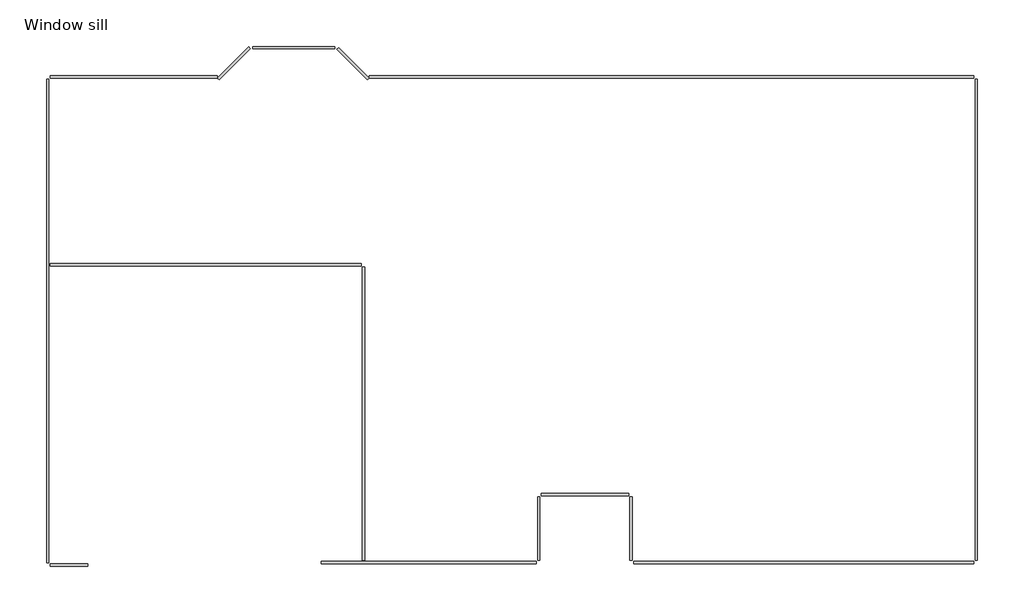
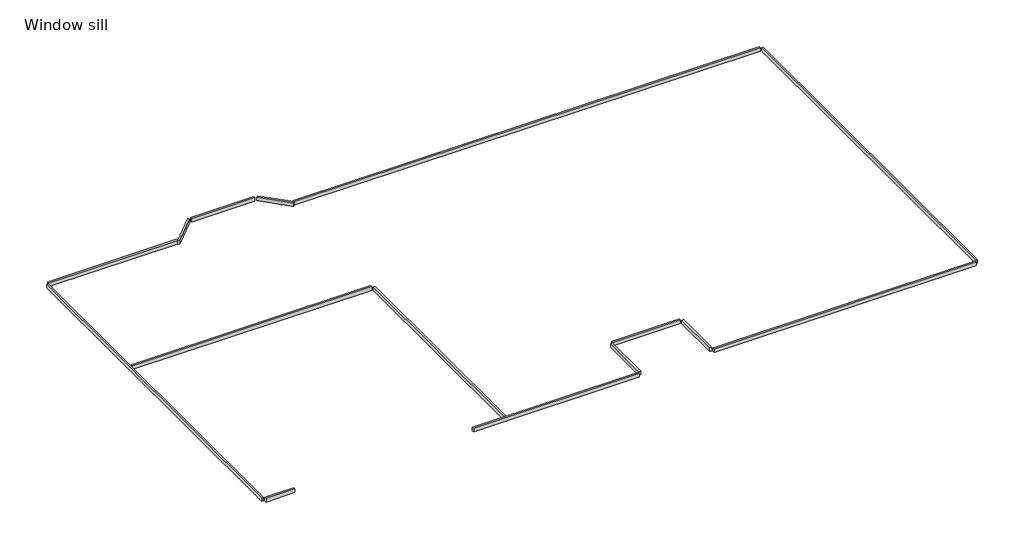
# One storey: 15 beams.
"""IFC4 building model written with IfcOpenShell, lengths in millimetres."""

import ifcopenshell
import ifcopenshell.guid

model = None  # the IFC model being written
_history = None  # IfcOwnerHistory: only IFC2X3 demands one
_inside = {}  # id of a spatial element -> (the spatial element, [elements in it])
_under = {}  # id of a project, library or spatial element -> (it, [spatial elements below it])
_declared = {}  # id of a project -> (the project, [libraries it declares])
_typed = {}  # id of a type object -> (the type object, [elements of that type])
_made_of = {}  # id of a material, layer set ... -> (it, [elements and type objects made of it])


def new_model(schema):
    """Start an empty IFC model of exactly this schema.

    Asked for "IFC4X3", IfcOpenShell would pick the latest addendum, in which some entities
    have other attributes; the version numbers below select the first issue.
    IFC2X3 requires an IfcOwnerHistory on every rooted entity: one is made here for all.
    """
    global model, _history
    if schema == "IFC4X3":
        model = ifcopenshell.file(schema_version=(4, 3, 0, 0))
    else:
        model = ifcopenshell.file(schema=schema)
    _inside.clear()
    _under.clear()
    _declared.clear()
    _typed.clear()
    _made_of.clear()
    _history = None
    if model.schema == "IFC2X3":
        org = make("IfcOrganization", Name="unknown")
        user = make(
            "IfcPersonAndOrganization",
            ThePerson=make("IfcPerson", FamilyName="unknown"),
            TheOrganization=org,
        )
        app = make(
            "IfcApplication",
            ApplicationDeveloper=org,
            Version="unknown",
            ApplicationFullName="unknown",
            ApplicationIdentifier="unknown",
        )
        _history = make(
            "IfcOwnerHistory",
            OwningUser=user,
            OwningApplication=app,
            ChangeAction="ADDED",
            CreationDate=0,
        )
    return model


def make(cls, **values):
    """One entity of the class cls with the attributes given. An attribute that is None is left unset."""
    return model.create_entity(
        cls, **{name: value for name, value in values.items() if value is not None}
    )


def rooted(cls, **values):
    """An entity with a GlobalId (a new one), such as an element, a storey or a relation."""
    return make(cls, GlobalId=ifcopenshell.guid.new(), OwnerHistory=_history, **values)


def si_unit(unit_type, name, prefix=None):
    """IfcSIUnit, for example si_unit("LENGTHUNIT", "METRE", prefix="MILLI")."""
    return make("IfcSIUnit", UnitType=unit_type, Prefix=prefix, Name=name)


def assignment(units):
    """IfcUnitAssignment: the units of a project."""
    return None if units is None else make("IfcUnitAssignment", Units=units)


def point(xyz):
    """IfcCartesianPoint."""
    return None if xyz is None else make("IfcCartesianPoint", Coordinates=xyz)


def direction(xyz):
    """IfcDirection."""
    return None if xyz is None else make("IfcDirection", DirectionRatios=xyz)


def frame(location, z_axis=None, x_axis=None):
    """IfcAxis2Placement3D, a coordinate frame: its origin and axes. An axis left out is left unset."""
    return make(
        "IfcAxis2Placement3D",
        Location=point(location),
        Axis=direction(z_axis),
        RefDirection=direction(x_axis),
    )


def origin():
    """The frame at (0, 0, 0) with its axes left unset."""
    return frame((0.0, 0.0, 0.0))


def place(relative_to, where):
    """IfcLocalPlacement: puts the frame where relative to a parent placement (None: the world)."""
    return make(
        "IfcLocalPlacement", PlacementRelTo=relative_to, RelativePlacement=where
    )


def context(
    kind, dimensions, precision=None, world=None, true_north=None, identifier=None
):
    """IfcGeometricRepresentationContext, for example the 3D "Model" context."""
    return make(
        "IfcGeometricRepresentationContext",
        ContextIdentifier=identifier,
        ContextType=kind,
        CoordinateSpaceDimension=dimensions,
        Precision=precision,
        WorldCoordinateSystem=world,
        TrueNorth=true_north,
    )


def project(units=None, contexts=None):
    """IfcProject with its units and contexts."""
    return rooted(
        "IfcProject",
        Name="project",
        RepresentationContexts=contexts,
        UnitsInContext=assignment(units),
    )


def spatial(cls, under=None, at=None, **own):
    """A site, building, storey or space (cls), placed at a placement, below another one or the project."""
    s = rooted(cls, ObjectPlacement=at, **own)
    if under is not None:
        _under.setdefault(under.id(), (under, []))[1].append(s)
    return s


def polyline(points):
    """IfcPolyline through the points."""
    return make("IfcPolyline", Points=[point(p) for p in points])


def outline(outer, holes=None, kind="AREA"):
    """IfcArbitraryClosedProfileDef: a profile drawn as a closed curve; with holes, ...WithVoids."""
    if holes is None:
        return make("IfcArbitraryClosedProfileDef", ProfileType=kind, OuterCurve=outer)
    return make(
        "IfcArbitraryProfileDefWithVoids",
        ProfileType=kind,
        OuterCurve=outer,
        InnerCurves=holes,
    )


def extrude(swept, where, along, depth):
    """IfcExtrudedAreaSolid: the profile swept, set in the frame where, extruded along a direction by depth."""
    return make(
        "IfcExtrudedAreaSolid",
        SweptArea=swept,
        Position=where,
        ExtrudedDirection=direction(along),
        Depth=depth,
    )


def shape(context_of_items, identifier, shape_type, items):
    """IfcShapeRepresentation: the items that make up one representation, for example the "Body"."""
    return make(
        "IfcShapeRepresentation",
        ContextOfItems=context_of_items,
        RepresentationIdentifier=identifier,
        RepresentationType=shape_type,
        Items=items,
    )


def source(mapping_origin, context_of_items, identifier, shape_type, items):
    """IfcRepresentationMap: a shape defined once, which mapped items show again and again."""
    return make(
        "IfcRepresentationMap",
        MappingOrigin=mapping_origin,
        MappedRepresentation=shape(context_of_items, identifier, shape_type, items),
    )


def transform(
    local_origin,
    x_axis=None,
    y_axis=None,
    z_axis=None,
    scale=None,
    scale2=None,
    scale3=None,
    uniform=True,
):
    """IfcCartesianTransformationOperator3D, or its non-uniform kind. x_axis, y_axis, z_axis: its Axis1, 2, 3."""
    if uniform:
        return make(
            "IfcCartesianTransformationOperator3D",
            Axis1=direction(x_axis),
            Axis2=direction(y_axis),
            LocalOrigin=point(local_origin),
            Scale=scale,
            Axis3=direction(z_axis),
        )
    return make(
        "IfcCartesianTransformationOperator3DnonUniform",
        Axis1=direction(x_axis),
        Axis2=direction(y_axis),
        LocalOrigin=point(local_origin),
        Scale=scale,
        Axis3=direction(z_axis),
        Scale2=scale2,
        Scale3=scale3,
    )


def mapped(mapping_source, mapping_target):
    """IfcMappedItem: shows the shape of a source again, moved by a transform."""
    return make(
        "IfcMappedItem", MappingSource=mapping_source, MappingTarget=mapping_target
    )


def made_of(thing, what):
    """Note that an element or type object is made of a material, layer set ...; save() writes the relation."""
    if what is not None:
        _made_of.setdefault(what.id(), (what, []))[1].append(thing)
    return thing


def element(
    cls,
    number,
    at=None,
    inside=None,
    cuts=None,
    type_object=None,
    material=None,
    context=None,
    identifier="Body",
    shape_type=None,
    held_by="IfcProductDefinitionShape",
    body=None,
    shapes=None,
    **own,
):
    """One element of the class cls, such as IfcWall. Its Tag is "e" and its number.

    at: its placement. inside: the storey or other place that contains it. cuts: it is an
    opening in that element (IfcRelVoidsElement). A single representation is given by context,
    identifier, shape_type and body (its items); several are given by shapes. held_by: the class
    of the entity that holds the representations. save() writes the other relations.
    """
    e = rooted(cls, Tag="e%d" % number, ObjectPlacement=at, **own)
    if body is not None:
        shapes = [shape(context, identifier, shape_type, body)]
    if shapes is not None:
        e.Representation = make(held_by, Representations=shapes)
    if inside is not None:
        _inside.setdefault(inside.id(), (inside, []))[1].append(e)
    if cuts is not None:
        rooted(
            "IfcRelVoidsElement", RelatingBuildingElement=cuts, RelatedOpeningElement=e
        )
    if type_object is not None:
        _typed.setdefault(type_object.id(), (type_object, []))[1].append(e)
    return made_of(e, material)


def aggregate(whole, parts):
    """IfcRelAggregates: a whole, such as a stair, and the parts it consists of."""
    return rooted("IfcRelAggregates", RelatingObject=whole, RelatedObjects=parts)


def save(model, path):
    """Write the relations noted so far, then the file.

    IfcRelAggregates (storeys below a building ...), IfcRelContainedInSpatialStructure (elements
    in a storey), IfcRelDefinesByType, IfcRelAssociatesMaterial and IfcRelDeclares: one each for
    every whole, place, type object, material and project.
    """
    for whole, parts in _under.values():
        aggregate(whole, parts)
    for where, things in _inside.values():
        rooted(
            "IfcRelContainedInSpatialStructure",
            RelatedElements=things,
            RelatingStructure=where,
        )
    for kind, things in _typed.values():
        rooted("IfcRelDefinesByType", RelatedObjects=things, RelatingType=kind)
    for what, things in _made_of.values():
        rooted("IfcRelAssociatesMaterial", RelatedObjects=things, RelatingMaterial=what)
    for by, libraries in _declared.values():
        rooted("IfcRelDeclares", RelatingContext=by, RelatedDefinitions=libraries)
    model.write(path)


def beam_717df711(model_context):
    return source(origin(), model_context, "Body", "SweptSolid", [
        extrude(outline(polyline([(1716.6789755, 25.4), (1716.6789755, -25.4), (-1777.9999994, -25.4), (-1777.9999994, 25.4), (1716.6789755, 25.4)])), frame((0.0, 0.0, -50.8), z_axis=(0.0, 0.0, 1.0), x_axis=(1.0, 0.0, 0.0)), (0.0, 0.0, 1.0), 101.6),
    ])


def beam_0fe92c09(model_context):
    return source(origin(), model_context, "Body", "SweptSolid", [
        extrude(outline(polyline([(431.690501, 25.4), (431.690501, -25.4), (-492.3733183, -25.4), (-492.3733183, 25.4), (431.690501, 25.4)])), frame((0.0, 0.0, -50.8), z_axis=(0.0, 0.0, 1.0), x_axis=(1.0, 0.0, 0.0)), (0.0, 0.0, 1.0), 101.6),
    ])


def beam_3500c81b(model_context):
    return source(origin(), model_context, "Body", "SweptSolid", [
        extrude(outline(polyline([(863.6, 25.4), (863.6, -25.4), (-845.1882072, -25.4), (-845.1882072, 25.4), (863.6, 25.4)])), frame((0.0, 0.0, -50.8), z_axis=(0.0, 0.0, 1.0), x_axis=(1.0, 0.0, 0.0)), (0.0, 0.0, 1.0), 101.6),
    ])


def beam_4e9e3d70(model_context):
    return source(origin(), model_context, "Body", "SweptSolid", [
        extrude(outline(polyline([(492.3733183, 25.4), (492.3733183, -25.4), (-405.6522938, -25.4), (-405.6522938, 25.4), (492.3733183, 25.4)])), frame((0.0, 0.0, -50.8), z_axis=(0.0, 0.0, 1.0), x_axis=(1.0, 0.0, 0.0)), (0.0, 0.0, 1.0), 101.6),
    ])


def beam_5a8d2df6(model_context):
    return source(origin(), model_context, "Body", "SweptSolid", [
        extrude(outline(polyline([(6349.9999994, 25.4), (6349.9999994, -25.4), (-6288.6789755, -25.4), (-6288.6789755, 25.4), (6349.9999994, 25.4)])), frame((0.0, 0.0, -50.8), z_axis=(0.0, 0.0, 1.0), x_axis=(1.0, 0.0, 0.0)), (0.0, 0.0, 1.0), 101.6),
    ])


def beam_8dd97a7c(model_context):
    return source(origin(), model_context, "Body", "SweptSolid", [
        extrude(outline(polyline([(5029.1999994, 25.4), (5029.1999994, -25.4), (-5029.1999994, -25.4), (-5029.1999994, 25.4), (5029.1999994, 25.4)])), frame((0.0, 0.0, -50.8), z_axis=(0.0, 0.0, 1.0), x_axis=(1.0, 0.0, 0.0)), (0.0, 0.0, 1.0), 101.6),
    ])


def beam_44bcd8c2(model_context):
    return source(origin(), model_context, "Body", "SweptSolid", [
        extrude(outline(polyline([(3555.9999994, 25.4), (3555.9999994, -25.4), (-3555.9999994, -25.4), (-3555.9999994, 25.4), (3555.9999994, 25.4)])), frame((0.0, 0.0, -50.8), z_axis=(0.0, 0.0, 1.0), x_axis=(1.0, 0.0, 0.0)), (0.0, 0.0, 1.0), 101.6),
    ])


def beam_ec20356b(model_context):
    return source(origin(), model_context, "Body", "SweptSolid", [
        extrude(outline(polyline([(660.3999994, 25.4), (660.3999994, -25.4), (-660.3999994, -25.4), (-660.3999994, 25.4), (660.3999994, 25.4)])), frame((0.0, 0.0, -50.8), z_axis=(0.0, 0.0, 1.0), x_axis=(1.0, 0.0, 0.0)), (0.0, 0.0, 1.0), 101.6),
    ])


def beam_17170791(model_context):
    return source(origin(), model_context, "Body", "SweptSolid", [
        extrude(outline(polyline([(914.3999994, 25.4), (914.3999994, -25.4), (-914.3999994, -25.4), (-914.3999994, 25.4), (914.3999994, 25.4)])), frame((0.0, 0.0, -50.8), z_axis=(0.0, 0.0, 1.0), x_axis=(1.0, 0.0, 0.0)), (0.0, 0.0, 1.0), 101.6),
    ])


def beam_5c93efd5(model_context):
    return source(origin(), model_context, "Body", "SweptSolid", [
        extrude(outline(polyline([(3063.8749994, 25.4), (3063.8749994, -25.4), (-3063.8749994, -25.4), (-3063.8749994, 25.4), (3063.8749994, 25.4)])), frame((0.0, 0.0, -50.8), z_axis=(0.0, 0.0, 1.0), x_axis=(1.0, 0.0, 0.0)), (0.0, 0.0, 1.0), 101.6),
    ])


def beam_4ff5e491(model_context):
    return source(origin(), model_context, "Body", "SweptSolid", [
        extrude(outline(polyline([(3248.0249994, 25.4), (3248.0249994, -25.4), (-3248.0249994, -25.4), (-3248.0249994, 25.4), (3248.0249994, 25.4)])), frame((0.0, 0.0, -50.8), z_axis=(0.0, 0.0, 1.0), x_axis=(1.0, 0.0, 0.0)), (0.0, 0.0, 1.0), 101.6),
    ])


def beam_8f11d8aa(model_context):
    return source(origin(), model_context, "Body", "SweptSolid", [
        extrude(outline(polyline([(5054.5999994, 25.4), (5054.5999994, -25.4), (-5054.5999994, -25.4), (-5054.5999994, 25.4), (5054.5999994, 25.4)])), frame((0.0, 0.0, -50.8), z_axis=(0.0, 0.0, 1.0), x_axis=(1.0, 0.0, 0.0)), (0.0, 0.0, 1.0), 101.6),
    ])


def beam_175a3536(model_context):
    return source(origin(), model_context, "Body", "SweptSolid", [
        extrude(outline(polyline([(2249.4875, 25.4), (2249.4875, -25.4), (-2249.4874994, -25.4), (-2249.4874994, 25.4), (2249.4875, 25.4)])), frame((0.0, 0.0, -50.8), z_axis=(0.0, 0.0, 1.0), x_axis=(1.0, 0.0, 0.0)), (0.0, 0.0, 1.0), 101.6),
    ])


def beam_ce158ae4(model_context):
    return source(origin(), model_context, "Body", "SweptSolid", [
        extrude(outline(polyline([(392.1124994, 25.4), (392.1124994, -25.4), (-392.1125, -25.4), (-392.1125, 25.4), (392.1124994, 25.4)])), frame((0.0, 0.0, -50.8), z_axis=(0.0, 0.0, 1.0), x_axis=(1.0, 0.0, 0.0)), (0.0, 0.0, 1.0), 101.6),
    ])


model = new_model("IFC4")

# Units and contexts
model_context = context("Model", 3, world=origin())
ifc_project = project(units=[si_unit("LENGTHUNIT", "METRE", prefix="MILLI")], contexts=[model_context])

# Site, building, storey
site = spatial("IfcSite", under=ifc_project)
building = spatial("IfcBuilding", under=site)
storey = spatial("IfcBuildingStorey", under=building, Name="Window sill", Elevation=1168.4)

# Beams
placement = place(None, origin())
beam_shape = beam_717df711(model_context)
element("IfcBeam", 1, ObjectType="Dimension Lumber : BLDG 6241 2X4\" TRUSS MEMBER", at=placement, inside=storey, context=model_context, shape_type="MappedRepresentation", body=[
    mapped(beam_shape, transform((-15921.614829, 5156.9284114, 1117.6), x_axis=(1.0, 0.0, 0.0), y_axis=(0.0, 1.0, 0.0), z_axis=(0.0, 0.0, 1.0))),
])
beam_2_shape = beam_0fe92c09(model_context)
element("IfcBeam", 2, ObjectType="Dimension Lumber : BLDG 6241 2X4\" TRUSS MEMBER", at=placement, inside=storey, context=model_context, shape_type="MappedRepresentation", body=[
    mapped(beam_2_shape, transform((-13838.814829, 5461.7284114, 1117.6), x_axis=(0.7071067811865481, 0.7071067811865468, 0.0), y_axis=(-0.7071067811865468, 0.7071067811865481, 0.0), z_axis=(0.0, 0.0, 1.0))),
])
beam_3_shape = beam_3500c81b(model_context)
element("IfcBeam", 3, ObjectType="Dimension Lumber : BLDG 6241 2X4\" TRUSS MEMBER", at=placement, inside=storey, context=model_context, shape_type="MappedRepresentation", body=[
    mapped(beam_3_shape, transform((-12619.614829, 5766.5284114, 1117.6), x_axis=(1.0, 0.0, 0.0), y_axis=(0.0, 1.0, 0.0), z_axis=(0.0, 0.0, 1.0))),
])
beam_4_shape = beam_4e9e3d70(model_context)
element("IfcBeam", 4, ObjectType="Dimension Lumber : BLDG 6241 2X4\" TRUSS MEMBER", at=placement, inside=storey, context=model_context, shape_type="MappedRepresentation", body=[
    mapped(beam_4_shape, transform((-11400.414829, 5461.7284114, 1117.6), x_axis=(0.7071067811865464, -0.7071067811865488, 0.0), y_axis=(0.7071067811865488, 0.7071067811865464, 0.0), z_axis=(0.0, 0.0, 1.0))),
])
beam_5_shape = beam_5a8d2df6(model_context)
element("IfcBeam", 5, ObjectType="Dimension Lumber : BLDG 6241 2X4\" TRUSS MEMBER", at=placement, inside=storey, context=model_context, shape_type="MappedRepresentation", body=[
    mapped(beam_5_shape, transform((-4745.614829, 5156.9284114, 1117.6), x_axis=(1.0, 0.0, 0.0), y_axis=(0.0, 1.0, 0.0), z_axis=(0.0, 0.0, 1.0))),
])
beam_6_shape = beam_8dd97a7c(model_context)
element("IfcBeam", 6, ObjectType="Dimension Lumber : BLDG 6241 2X4\" TRUSS MEMBER", at=placement, inside=storey, context=model_context, shape_type="MappedRepresentation", body=[
    mapped(beam_6_shape, transform((1655.185171, 76.9284114, 1117.6), x_axis=(0.0, -1.0, 0.0), y_axis=(1.0, 0.0, 0.0), z_axis=(0.0, 0.0, 1.0))),
])
beam_7_shape = beam_44bcd8c2(model_context)
element("IfcBeam", 7, ObjectType="Dimension Lumber : BLDG 6241 2X4\" TRUSS MEMBER", at=placement, inside=storey, context=model_context, shape_type="MappedRepresentation", body=[
    mapped(beam_7_shape, transform((-1951.614829, -5003.0715886, 1117.6), x_axis=(-1.0, 0.0, 0.0), y_axis=(0.0, -1.0, 0.0), z_axis=(0.0, 0.0, 1.0))),
])
beam_8_shape = beam_ec20356b(model_context)
element("IfcBeam", 8, ObjectType="Dimension Lumber : BLDG 6241 2X4\" TRUSS MEMBER", at=placement, inside=storey, context=model_context, shape_type="MappedRepresentation", body=[
    mapped(beam_8_shape, transform((-5558.414829, -4291.8715886, 1117.6), x_axis=(0.0, 1.0, 0.0), y_axis=(-1.0, 0.0, 0.0), z_axis=(0.0, 0.0, 1.0))),
])
element("IfcBeam", 9, ObjectType="Dimension Lumber : BLDG 6241 2X4\" TRUSS MEMBER", at=placement, inside=storey, context=model_context, shape_type="MappedRepresentation", body=[
    mapped(beam_8_shape, transform((-7488.814829, -4291.8715886, 1117.6), x_axis=(0.0, -1.0, 0.0), y_axis=(1.0, 0.0, 0.0), z_axis=(0.0, 0.0, 1.0))),
])
beam_9_shape = beam_17170791(model_context)
element("IfcBeam", 10, ObjectType="Dimension Lumber : BLDG 6241 2X4\" TRUSS MEMBER", at=placement, inside=storey, context=model_context, shape_type="MappedRepresentation", body=[
    mapped(beam_9_shape, transform((-6523.614829, -3580.6715886, 1117.6), x_axis=(-1.0, 0.0, 0.0), y_axis=(0.0, -1.0, 0.0), z_axis=(0.0, 0.0, 1.0))),
])
beam_10_shape = beam_5c93efd5(model_context)
element("IfcBeam", 11, ObjectType="Dimension Lumber : BLDG 6241 2X4\" TRUSS MEMBER", at=placement, inside=storey, context=model_context, shape_type="MappedRepresentation", body=[
    mapped(beam_10_shape, transform((-11152.764829, -1888.3965886, 1117.6), x_axis=(0.0, 1.0, 0.0), y_axis=(-1.0, 0.0, 0.0), z_axis=(0.0, 0.0, 1.0))),
])
beam_11_shape = beam_4ff5e491(model_context)
element("IfcBeam", 12, ObjectType="Dimension Lumber : BLDG 6241 2X4\" TRUSS MEMBER", at=placement, inside=storey, context=model_context, shape_type="MappedRepresentation", body=[
    mapped(beam_11_shape, transform((-14451.589829, 1226.2784114, 1117.6), x_axis=(-1.0, 0.0, 0.0), y_axis=(0.0, -1.0, 0.0), z_axis=(0.0, 0.0, 1.0))),
])
beam_12_shape = beam_8f11d8aa(model_context)
element("IfcBeam", 13, ObjectType="Dimension Lumber : BLDG 6241 2X4\" TRUSS MEMBER", at=placement, inside=storey, context=model_context, shape_type="MappedRepresentation", body=[
    mapped(beam_12_shape, transform((-17750.414829, 51.5284114, 1117.6), x_axis=(0.0, 1.0, 0.0), y_axis=(-1.0, 0.0, 0.0), z_axis=(0.0, 0.0, 1.0))),
])
beam_13_shape = beam_175a3536(model_context)
element("IfcBeam", 14, ObjectType="Dimension Lumber : BLDG 6241 2X4\" TRUSS MEMBER", at=placement, inside=storey, context=model_context, shape_type="MappedRepresentation", body=[
    mapped(beam_13_shape, transform((-9789.102329, -5003.0715886, 1117.6), x_axis=(-1.0, 0.0, 0.0), y_axis=(0.0, -1.0, 0.0), z_axis=(0.0, 0.0, 1.0))),
])
beam_14_shape = beam_ce158ae4(model_context)
element("IfcBeam", 15, ObjectType="Dimension Lumber : BLDG 6241 2X4\" TRUSS MEMBER", at=placement, inside=storey, context=model_context, shape_type="MappedRepresentation", body=[
    mapped(beam_14_shape, transform((-17307.502329, -5053.8715886, 1117.6), x_axis=(-1.0, 0.0, 0.0), y_axis=(0.0, -1.0, 0.0), z_axis=(0.0, 0.0, 1.0))),
])

save(model, "model.ifc")

# Revit data of these elements
# Type "Dimension Lumber : BLDG 6241 2X4\" TRUSS MEMBER"
#   Assembly Code = "B10"
#   A = 0.273472 SF
#   Length [instance default] = 5' - 0"
#   b = 0' - 2"
#   d = 0' - 4"
#   Structural Material [instance default] = Softwood, Lumber
# Elements 1, 2, 3, 4, 5, 6, 7, 8, 9, 10, 11, 12, 13, 14, 15 (IfcBeam, "Dimension Lumber : BLDG 6241 2X4\" TRUSS MEMBER")
#   Comments = ""
#   Structural Material = Softwood, Lumber
#   Phase Created = New Construction
#   Materials on its faces: "Softwood, Lumber"
# Materials
#   "Softwood, Lumber": class "Wood", colour RGB 223 192 134, transparency 0, Description = "Pinus Echinata", Cost = 0
